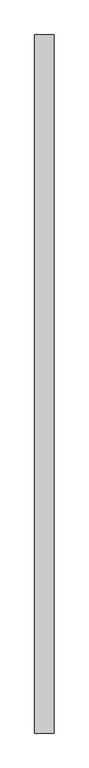
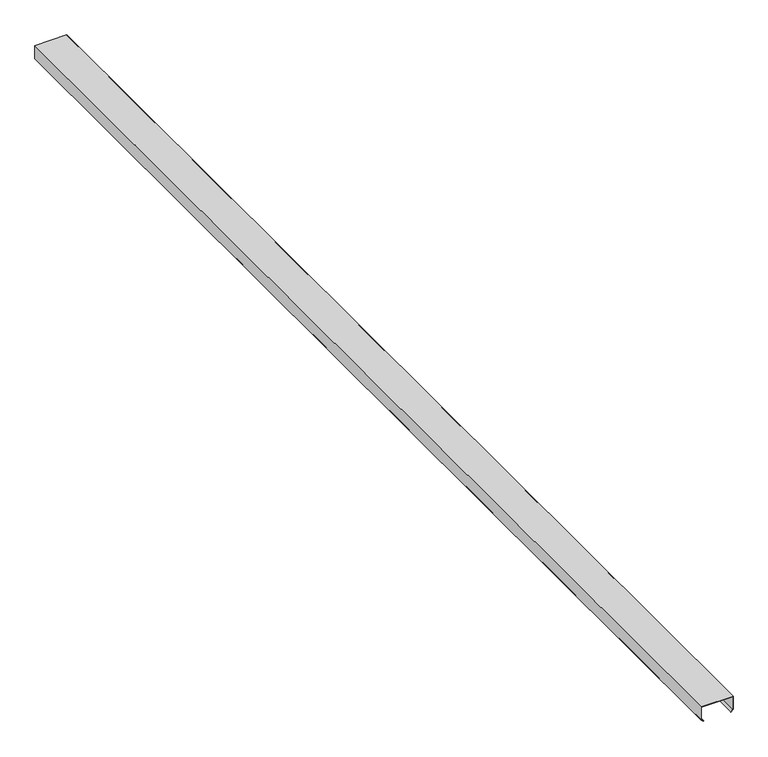
"""IFC4 building model written with IfcOpenShell, lengths in millimetres: proxy geometry, Generic Models 7:Generic Models 1:1:Generic Models 1:1 : Generic Models 7:Generic Models 1:337419:24 : Generic Models 7:Generic Models 1:1:Generic Models 1:1 : Generic Models 7:Generic Models 1:337419:306201."""

from ifc_helpers import new_model, si_unit, frame, origin, place, context, project, spatial, polyline, outline, extrude, source, transform, mapped, element, save


def generic_models_f74ef017(model_context):
    return source(origin(), model_context, "Body", "SweptSolid", [
        extrude(outline(polyline([(6128.940625, 560556.1617239), (6128.940625, 560352.9617239), (6040.040625, 560352.9617239), (6027.7955211, 560367.5548705), (6029.9236883, 560369.3406148), (6041.336086, 560355.7398489), (6126.1625, 560355.7398489), (6126.1625, 560553.3835989), (6041.336086, 560553.3835989), (6029.9236883, 560539.7828329), (6027.7955211, 560541.5685772), (6040.040625, 560556.1617239), (6128.940625, 560556.1617239)])), frame((0.0, -579000.6913841, 0.0), z_axis=(0.0, 1.0, 0.0), x_axis=(0.0, 0.0, 1.0)), (0.0, 0.0, 1.0), 7315.2),
    ])


if __name__ == "__main__":
    model = new_model("IFC4")
    model_context = context("Model", 3, world=origin())
    ifc_project = project(units=[si_unit("LENGTHUNIT", "METRE", prefix="MILLI")], contexts=[model_context])
    site = spatial("IfcSite", under=ifc_project)
    building = spatial("IfcBuilding", under=site)
    placement = place(None, origin())
    generic_models_shape = generic_models_f74ef017(model_context)
    element("IfcBuildingElementProxy", 1, Name="Generic Models 7:Generic Models 1:1:Generic Models 1:1 : Generic Models 7:Generic Models 1:337419:24 : Generic Models 7:Generic Models 1:1:Generic Models 1:1 : Generic Models 7:Generic Models 1:337419:306201", ObjectType="Generic Models 7:Generic Models 1:1:Generic Models 1:1 : Generic Models 7:Generic Models 1:337419:24 : Generic Models 7:Generic Models 1:1:Generic Models 1:1 : Generic Models 7:Generic Models 1:337419:306201", at=placement, inside=building, context=model_context, shape_type="MappedRepresentation", body=[
        mapped(generic_models_shape, transform((0.0, 0.0, 0.0), x_axis=(1.0, 0.0, 0.0), y_axis=(0.0, 1.0, 0.0), z_axis=(0.0, 0.0, 1.0))),
    ])
    save(model, "model.ifc")

# Revit data of these elements
# Type "Generic Models 7:Generic Models 1:1:Generic Models 1:1 : Generic Models 7:Generic Models 1:337419:24 : Generic Models 7:Generic Models 1:1:Generic Models 1:1 : Generic Models 7:Generic Models 1:337419:306201"
#   NameOverride = "Generic Models 7:Generic Models 1:1:Generic Models 1:1 : Generic Models 7:Generic Models 1:337419:306201"
#   ObjectTypeOverride = "Generic Models 1:1 : Generic Models 7:Generic Models 1:337419"
#   Reference = "Generic Models 1"
#   Tag = "306201"
# Element 1 (IfcBuildingElementProxy, "Generic Models 7:Generic Models 1:1:Generic Models 1:1 : Generic Models 7:Generic Models 1:337419:24 : Generic Models 7:Generic Models 1:1:Generic Models 1:1 : Generic Models 7:Generic Models 1:337419:306201")
#   Materials on its faces: "GALVANIZED 'CEE' SECTION (8.0x3.5C - SEE STRUCT. DWGS)"
# Materials
#   "GALVANIZED 'CEE' SECTION (8.0x3.5C - SEE STRUCT. DWGS)": class "Unassigned", colour RGB 210 209 208, transparency 0, Keynote = "M05121300.02", Cost = 0
